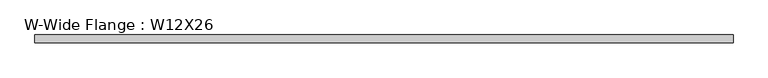
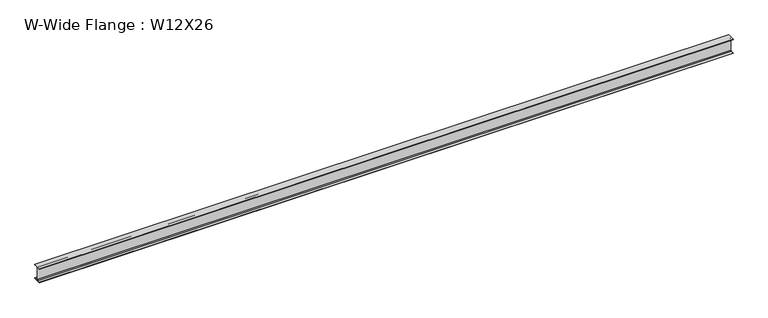
"""IFC4 building model written with IfcOpenShell, lengths in millimetres: beam geometry, W-Wide Flange : W12X26."""

from ifc_helpers import new_model, si_unit, point, frame, frame_2d, origin, place, context, project, spatial, polyline, circle_curve, trimmed, segment, composite_curve, outline, extrude, source, transform, mapped, element, save


def w_wide_flange_w12x26_f0aa8a0b(model_context):
    return source(origin(), model_context, "Body", "SweptSolid", [
        extrude(outline(composite_curve([segment(polyline([(82.4011719, -145.5539063), (82.4011719, -155.178125), (-82.4011719, -155.178125), (-82.4011719, -145.5539063), (-20.2902344, -145.5539063)]), True, "CONTINUOUS"), segment(trimmed(circle_curve(frame_2d((-20.2902344, -128.190625)), 17.3632812), [point((-20.2902344, -145.5539063))], [point((-2.9269531, -128.190625))], True, "CARTESIAN"), True, "CONTINUOUS"), segment(polyline([(-2.9269531, -128.190625), (-2.9269531, 128.190625)]), True, "CONTINUOUS"), segment(trimmed(circle_curve(frame_2d((-20.2902344, 128.190625)), 17.3632812), [point((-2.9269531, 128.190625))], [point((-20.2902344, 145.5539062))], True, "CARTESIAN"), True, "CONTINUOUS"), segment(polyline([(-20.2902344, 145.5539062), (-82.4011719, 145.5539062), (-82.4011719, 155.178125), (82.4011719, 155.178125), (82.4011719, 145.5539062), (20.2902344, 145.5539062)]), True, "CONTINUOUS"), segment(trimmed(circle_curve(frame_2d((20.2902344, 128.190625)), 17.3632812), [point((20.2902344, 145.5539062))], [point((2.9269531, 128.190625))], True, "CARTESIAN"), True, "CONTINUOUS"), segment(polyline([(2.9269531, 128.190625), (2.9269531, -128.190625)]), True, "CONTINUOUS"), segment(trimmed(circle_curve(frame_2d((20.2902344, -128.190625)), 17.3632812), [point((2.9269531, -128.190625))], [point((20.2902344, -145.5539063))], True, "CARTESIAN"), True, "CONTINUOUS"), segment(polyline([(20.2902344, -145.5539063), (82.4011719, -145.5539063)]), True, "CONTINUOUS")], self_intersect=False)), frame((-7315.2, 0.0, 0.0), z_axis=(1.0, 0.0, 0.0), x_axis=(0.0, 1.0, 0.0)), (0.0, 0.0, 1.0), 14482.9889312),
    ])


if __name__ == "__main__":
    model = new_model("IFC4")
    model_context = context("Model", 3, world=origin())
    ifc_project = project(units=[si_unit("LENGTHUNIT", "METRE", prefix="MILLI")], contexts=[model_context])
    site = spatial("IfcSite", under=ifc_project)
    building = spatial("IfcBuilding", under=site)
    placement = place(None, origin())
    w_wide_flange_w12x26_shape = w_wide_flange_w12x26_f0aa8a0b(model_context)
    element("IfcBeam", 1, ObjectType="W-Wide Flange : W12X26", at=placement, inside=building, context=model_context, shape_type="MappedRepresentation", body=[
        mapped(w_wide_flange_w12x26_shape, transform((0.0, 0.0, 0.0), x_axis=(1.0, 0.0, 0.0), y_axis=(0.0, 1.0, 0.0), z_axis=(0.0, 0.0, 1.0))),
    ])
    save(model, "model.ifc")

# Revit data of these elements
# Type "W-Wide Flange : W12X26"
#   Assembly Code = "B10"
#   Start Extension Calculation [instance default] = 10' - 0"
#   Start Extension [instance default] = -0' - 0 1/2"
#   End Extension Calculation [instance default] = 10' - 0"
#   End Extension [instance default] = -0' - 0 1/2"
#   A = 0.053125 SF
#   Length [instance default] = 5' - 0"
#   W = 26
#   bf = 0' - 6 125/256"
#   d = 1' - 0 7/32"
#   k = 0' - 1 1/16"
#   k2 = 0' - 0 175/256"
#   tf = 0' - 0 97/256"
#   tw = 0' - 0 59/256"
#   Beam Material [instance default] = Metal - Steel - ASTM A992
# Element 1 (IfcBeam, "W-Wide Flange : W12X26")
#   Materials on its faces: "Metal - Steel - ASTM A992"
# Materials
#   "Metal - Steel - ASTM A992": class "Metal", colour RGB 199 199 199, transparency 0
